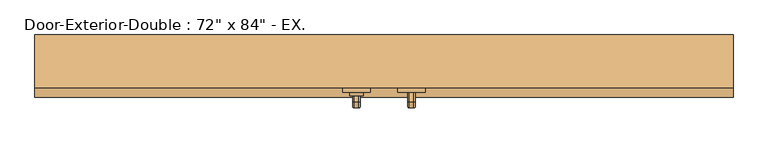
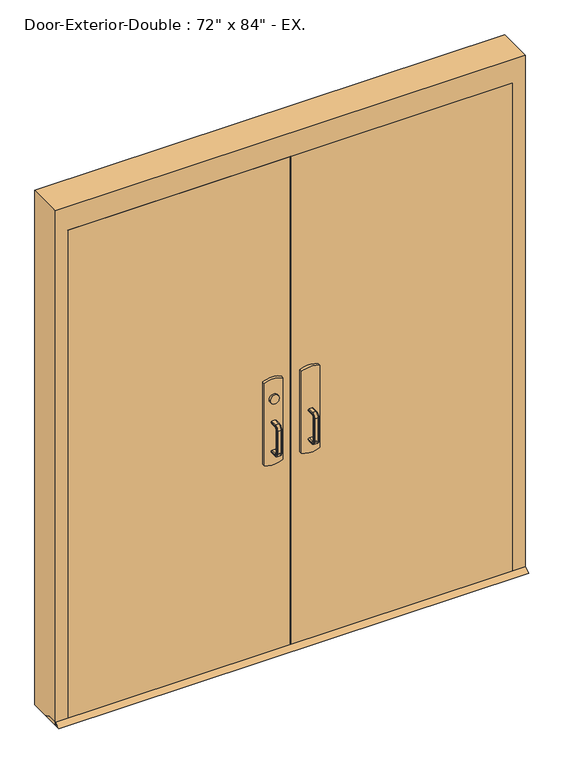
"""IFC4 building model written with IfcOpenShell, lengths in millimetres: door geometry."""

from ifc_helpers import new_model, si_unit, point, frame, frame_2d, origin, place, context, project, spatial, polyline, circle_curve, ellipse_curve, trimmed, segment, composite_curve, outline, extrude, faceted_brep, source, transform, mapped, element, save
from ifc_brep_helpers import plane_surface, cylinder_surface, revolved_surface, advanced_brep


def door_c05566ca(model_context):
    return source(origin(), model_context, "Body", "SolidModel", [
        extrude(outline(polyline([(-575.7333333, -15.875), (-76.2, -15.875), (-76.2, -22.225), (-575.7333333, -22.225), (-575.7333333, -15.875)])), frame((0.0, 0.0, 990.6), z_axis=(0.0, 0.0, 1.0), x_axis=(1.0, 0.0, 0.0)), (0.0, 0.0, 1.0), 50.8),
        advanced_brep(
        [(-12.7, -22.225, 1041.4), (-12.7, -22.225, 990.6), (-76.2, -22.225, 990.6), (-825.5, -22.225, 990.6), (-825.5, -22.225, 1041.4), (-76.2, -22.225, 1041.4), (-825.5, -53.975, 1041.4), (-825.5, -53.975, 990.6), (-76.2, -53.975, 990.6), (-76.2, -53.975, 927.1), (-57.15, -53.975, 908.05), (-31.75, -53.975, 908.05), (-12.7, -53.975, 927.1), (-12.7, -53.975, 1104.9), (-31.75, -53.975, 1123.95), (-57.15, -53.975, 1123.95), (-76.2, -53.975, 1104.9), (-76.2, -53.975, 1041.4), (-76.2, -25.4002467, 1041.4), (-12.7, -25.4002467, 1041.4), (-12.7, -30.4104269, 1104.9), (-12.7, -30.4104269, 927.1), (-12.7, -25.4002467, 990.6), (-76.2, -25.4002467, 990.6), (-76.2, -30.4104269, 1104.9), (-76.2, -30.4104269, 927.1), (-31.75, -31.913481, 1123.95), (-57.15, -31.913481, 1123.95), (-57.15, -31.913481, 908.05), (-31.75, -31.913481, 908.05)],
        [
            (0, 1),
            (1, 2),
            (2, 3),
            (3, 4),
            (4, 5),
            (5, 0),
            (6, 7),
            (7, 8),
            (8, 9),
            (9, 10, circle_curve(frame((-57.15, -53.975, 927.1), z_axis=(0.0, -1.0, 0.0), x_axis=(-1.0, 0.0, 0.0)), 19.05)),
            (10, 11),
            (11, 12, circle_curve(frame((-31.75, -53.975, 927.1), z_axis=(0.0, -1.0, 0.0), x_axis=(-1.0, 0.0, 0.0)), 19.05)),
            (12, 13),
            (13, 14, circle_curve(frame((-31.75, -53.975, 1104.9), z_axis=(0.0, -1.0, 0.0), x_axis=(-1.0, 0.0, 0.0)), 19.05)),
            (14, 15),
            (15, 16, circle_curve(frame((-57.15, -53.975, 1104.9), z_axis=(0.0, -1.0, 0.0), x_axis=(-1.0, 0.0, 0.0)), 19.05)),
            (16, 17),
            (17, 6),
            (4, 6),
            (17, 18),
            (18, 19),
            (19, 0),
            (19, 20),
            (20, 13),
            (12, 21),
            (21, 22),
            (22, 1),
            (7, 3),
            (22, 23),
            (23, 8),
            (16, 24),
            (24, 18),
            (23, 25),
            (25, 9),
            (14, 26),
            (26, 27),
            (27, 15),
            (10, 28),
            (28, 29),
            (29, 11),
            (25, 28, ellipse_curve(frame((-57.15, -30.4104269, 927.1), z_axis=(0.0, -0.9969018152893365, 0.07865602756830282), x_axis=(0.0, 0.07865602756830208, 0.9969018152893365)), 19.1092038, 19.05)),
            (27, 24, ellipse_curve(frame((-57.15, -30.4104269, 1104.9), z_axis=(0.0, -0.9969018152893376, -0.07865602756828934), x_axis=(0.0, 0.078656027568288, -0.9969018152893377)), 19.1092038, 19.05)),
            (20, 26, ellipse_curve(frame((-31.75, -30.4104269, 1104.9), z_axis=(0.0, -0.9969018152893376, -0.07865602756828934), x_axis=(0.0, 0.078656027568288, -0.9969018152893377)), 19.1092038, 19.05)),
            (29, 21, ellipse_curve(frame((-31.75, -30.4104269, 927.1), z_axis=(0.0, -0.9969018152893365, 0.07865602756830282), x_axis=(0.0, 0.07865602756830208, 0.9969018152893365)), 19.1092038, 19.05)),
        ],
        [
            plane_surface(frame((-12.7, -22.225, 1041.4), z_axis=(0.0, 1.0, 0.0), x_axis=(1.0, 0.0, 0.0))),
            plane_surface(frame((-12.7, -53.975, 1041.4), z_axis=(0.0, -1.0, 0.0), x_axis=(-1.0, 0.0, 0.0))),
            plane_surface(frame((-825.5, -22.225, 1041.4), z_axis=(0.0, 0.0, 1.0), x_axis=(0.0, -1.0, 0.0))),
            plane_surface(frame((-12.7, -22.225, 1041.4), z_axis=(1.0, 0.0, 0.0), x_axis=(0.0, -1.0, 0.0))),
            plane_surface(frame((-12.7, -22.225, 990.6), z_axis=(0.0, 0.0, -1.0), x_axis=(0.0, -1.0, 0.0))),
            plane_surface(frame((-825.5, -22.225, 990.6), z_axis=(-1.0, 0.0, 0.0), x_axis=(0.0, -1.0, 0.0))),
            plane_surface(frame((-76.2, -25.4002467, 927.1), z_axis=(-1.0, 0.0, 0.0), x_axis=(0.0, -1.0, 0.0))),
            plane_surface(frame((-57.15, -25.4002467, 1123.95), z_axis=(0.0, 0.0, 1.0), x_axis=(0.0, -1.0, 0.0))),
            plane_surface(frame((-31.75, -25.4002467, 908.05), z_axis=(0.0, 0.0, -1.0), x_axis=(0.0, -1.0, 0.0))),
            cylinder_surface(frame((-57.15, -53.975, 927.1), z_axis=(0.0, 1.0, 0.0), x_axis=(-1.0, 0.0, 0.0)), 19.05),
            cylinder_surface(frame((-57.15, -53.975, 1104.9), z_axis=(0.0, 1.0, 0.0), x_axis=(-1.0, 0.0, 0.0)), 19.05),
            cylinder_surface(frame((-31.75, -53.975, 1104.9), z_axis=(0.0, 1.0, 0.0), x_axis=(-1.0, 0.0, 0.0)), 19.05),
            cylinder_surface(frame((-31.75, -53.975, 927.1), z_axis=(0.0, 1.0, 0.0), x_axis=(-1.0, 0.0, 0.0)), 19.05),
            plane_surface(frame((-76.2, -25.4002467, 1041.4), z_axis=(0.0, 0.9969018152893376, 0.07865602756828934), x_axis=(1.0, 0.0, 0.0))),
            plane_surface(frame((-76.2, -31.913481, 908.05), z_axis=(0.0, 0.9969018152893365, -0.07865602756830282), x_axis=(1.0, 0.0, 0.0))),
        ],
        [
            (0, [[1, 2, 3, 4, 5, 6]]),
            (1, [[7, 8, 9, 10, 11, 12, 13, 14, 15, 16, 17, 18]]),
            (2, [[19, -18, 20, 21, 22, -6, -5]]),
            (3, [[-1, -22, 23, 24, -13, 25, 26, 27]]),
            (4, [[28, -3, -2, -27, 29, 30, -8]]),
            (5, [[-4, -28, -7, -19]]),
            (6, [[-17, 31, 32, -20]]),
            (6, [[-9, -30, 33, 34]]),
            (7, [[-15, 35, 36, 37]]),
            (8, [[-11, 38, 39, 40]]),
            (9, [[-10, -34, 41, -38]]),
            (10, [[-16, -37, 42, -31]]),
            (11, [[-14, -24, 43, -35]]),
            (12, [[-12, -40, 44, -25]]),
            (13, [[-21, -32, -42, -36, -43, -23]]),
            (14, [[-26, -44, -39, -41, -33, -29]]),
        ],
    ),
        extrude(outline(polyline([(-98.425, 12.7), (-53.975, 12.7), (-28.575, 0.0), (-123.825, 0.0), (-98.425, 12.7)])), frame((-965.2, 0.0, 0.0), z_axis=(1.0, 0.0, 0.0), x_axis=(0.0, 1.0, 0.0)), (0.0, 0.0, 1.0), 1930.4),
        extrude(outline(polyline([(575.7333333, -15.875), (575.7333333, -22.225), (76.2, -22.225), (76.2, -15.875), (575.7333333, -15.875)])), frame((0.0, 0.0, 990.6), z_axis=(0.0, 0.0, 1.0), x_axis=(1.0, 0.0, 0.0)), (0.0, 0.0, 1.0), 50.8),
        advanced_brep(
        [(12.7, -22.225, 1041.4), (76.2, -22.225, 1041.4), (825.5, -22.225, 1041.4), (825.5, -22.225, 990.6), (76.2, -22.225, 990.6), (12.7, -22.225, 990.6), (825.5, -53.975, 1041.4), (76.2, -53.975, 1041.4), (76.2, -53.975, 1104.9), (57.15, -53.975, 1123.95), (31.75, -53.975, 1123.95), (12.7, -53.975, 1104.9), (12.7, -53.975, 927.1), (31.75, -53.975, 908.05), (57.15, -53.975, 908.05), (76.2, -53.975, 927.1), (76.2, -53.975, 990.6), (825.5, -53.975, 990.6), (12.7, -25.4002467, 1041.4), (76.2, -25.4002467, 1041.4), (12.7, -25.4002467, 990.6), (12.7, -30.4104269, 927.1), (12.7, -30.4104269, 1104.9), (76.2, -25.4002467, 990.6), (76.2, -30.4104269, 1104.9), (76.2, -30.4104269, 927.1), (57.15, -31.913481, 1123.95), (31.75, -31.913481, 1123.95), (31.75, -31.913481, 908.05), (57.15, -31.913481, 908.05)],
        [
            (0, 1),
            (1, 2),
            (2, 3),
            (3, 4),
            (4, 5),
            (5, 0),
            (6, 7),
            (7, 8),
            (8, 9, circle_curve(frame((57.15, -53.975, 1104.9), z_axis=(0.0, -1.0, 0.0), x_axis=(1.0, 0.0, 0.0)), 19.05)),
            (9, 10),
            (10, 11, circle_curve(frame((31.75, -53.975, 1104.9), z_axis=(0.0, -1.0, 0.0), x_axis=(1.0, 0.0, 0.0)), 19.05)),
            (11, 12),
            (12, 13, circle_curve(frame((31.75, -53.975, 927.1), z_axis=(0.0, -1.0, 0.0), x_axis=(1.0, 0.0, 0.0)), 19.05)),
            (13, 14),
            (14, 15, circle_curve(frame((57.15, -53.975, 927.1), z_axis=(0.0, -1.0, 0.0), x_axis=(1.0, 0.0, 0.0)), 19.05)),
            (15, 16),
            (16, 17),
            (17, 6),
            (0, 18),
            (18, 19),
            (19, 7),
            (6, 2),
            (5, 20),
            (20, 21),
            (21, 12),
            (11, 22),
            (22, 18),
            (16, 23),
            (23, 20),
            (3, 17),
            (19, 24),
            (24, 8),
            (15, 25),
            (25, 23),
            (9, 26),
            (26, 27),
            (27, 10),
            (13, 28),
            (28, 29),
            (29, 14),
            (29, 25, ellipse_curve(frame((57.15, -30.4104269, 927.1), z_axis=(0.0, -0.9969018152893365, 0.07865602756830282), x_axis=(0.0, 0.07865602756830208, 0.9969018152893365)), 19.1092038, 19.05)),
            (24, 26, ellipse_curve(frame((57.15, -30.4104269, 1104.9), z_axis=(0.0, -0.9969018152893376, -0.07865602756828934), x_axis=(0.0, 0.078656027568288, -0.9969018152893377)), 19.1092038, 19.05)),
            (27, 22, ellipse_curve(frame((31.75, -30.4104269, 1104.9), z_axis=(0.0, -0.9969018152893376, -0.07865602756828934), x_axis=(0.0, 0.078656027568288, -0.9969018152893377)), 19.1092038, 19.05)),
            (21, 28, ellipse_curve(frame((31.75, -30.4104269, 927.1), z_axis=(0.0, -0.9969018152893365, 0.07865602756830282), x_axis=(0.0, 0.07865602756830208, 0.9969018152893365)), 19.1092038, 19.05)),
        ],
        [
            plane_surface(frame((12.7, -22.225, 1041.4), z_axis=(0.0, 1.0, 0.0), x_axis=(-1.0, 0.0, 0.0))),
            plane_surface(frame((12.7, -53.975, 1041.4), z_axis=(0.0, -1.0, 0.0), x_axis=(1.0, 0.0, 0.0))),
            plane_surface(frame((825.5, -22.225, 1041.4), z_axis=(0.0, 0.0, 1.0), x_axis=(0.0, -1.0, 0.0))),
            plane_surface(frame((12.7, -22.225, 1041.4), z_axis=(-1.0, 0.0, 0.0), x_axis=(0.0, -1.0, 0.0))),
            plane_surface(frame((12.7, -22.225, 990.6), z_axis=(0.0, 0.0, -1.0), x_axis=(0.0, -1.0, 0.0))),
            plane_surface(frame((825.5, -22.225, 990.6), z_axis=(1.0, 0.0, 0.0), x_axis=(0.0, -1.0, 0.0))),
            plane_surface(frame((76.2, -25.4002467, 927.1), z_axis=(1.0, 0.0, 0.0), x_axis=(0.0, -1.0, 0.0))),
            plane_surface(frame((57.15, -25.4002467, 1123.95), z_axis=(0.0, 0.0, 1.0), x_axis=(0.0, -1.0, 0.0))),
            plane_surface(frame((31.75, -25.4002467, 908.05), z_axis=(0.0, 0.0, -1.0), x_axis=(0.0, -1.0, 0.0))),
            cylinder_surface(frame((57.15, -53.975, 927.1), z_axis=(0.0, 1.0, 0.0), x_axis=(1.0, 0.0, 0.0)), 19.05),
            cylinder_surface(frame((57.15, -53.975, 1104.9), z_axis=(0.0, 1.0, 0.0), x_axis=(1.0, 0.0, 0.0)), 19.05),
            cylinder_surface(frame((31.75, -53.975, 1104.9), z_axis=(0.0, 1.0, 0.0), x_axis=(1.0, 0.0, 0.0)), 19.05),
            cylinder_surface(frame((31.75, -53.975, 927.1), z_axis=(0.0, 1.0, 0.0), x_axis=(1.0, 0.0, 0.0)), 19.05),
            plane_surface(frame((76.2, -25.4002467, 1041.4), z_axis=(0.0, 0.9969018152893376, 0.07865602756828934), x_axis=(-1.0, 0.0, 0.0))),
            plane_surface(frame((76.2, -31.913481, 908.05), z_axis=(0.0, 0.9969018152893365, -0.07865602756830282), x_axis=(-1.0, 0.0, 0.0))),
        ],
        [
            (0, [[1, 2, 3, 4, 5, 6]]),
            (1, [[7, 8, 9, 10, 11, 12, 13, 14, 15, 16, 17, 18]]),
            (2, [[-2, -1, 19, 20, 21, -7, 22]]),
            (3, [[23, 24, 25, -12, 26, 27, -19, -6]]),
            (4, [[-17, 28, 29, -23, -5, -4, 30]]),
            (5, [[-22, -18, -30, -3]]),
            (6, [[-21, 31, 32, -8]]),
            (6, [[33, 34, -28, -16]]),
            (7, [[35, 36, 37, -10]]),
            (8, [[38, 39, 40, -14]]),
            (9, [[-40, 41, -33, -15]]),
            (10, [[-32, 42, -35, -9]]),
            (11, [[-37, 43, -26, -11]]),
            (12, [[-25, 44, -38, -13]]),
            (13, [[-27, -43, -36, -42, -31, -20]]),
            (14, [[-29, -34, -41, -39, -44, -24]]),
        ],
    ),
        advanced_brep(
        [(66.2, -111.125, 1017.190625), (69.771875, -111.125, 1020.7625), (82.628125, -111.125, 1020.7625), (86.2, -111.125, 1017.190625), (86.2, -111.125, 1014.8090406), (82.6284594, -111.125, 1011.2375), (69.771875, -111.125, 1011.2375), (66.2, -111.125, 1014.809375), (66.2, -111.125, 887.809375), (66.2, -111.125, 890.190625), (69.771875, -111.125, 893.7625), (82.6284594, -111.125, 893.7625), (86.2, -111.125, 890.1909594), (86.2, -111.125, 887.809375), (82.628125, -111.125, 884.2375), (69.771875, -111.125, 884.2375), (66.2, -136.525, 1014.809375), (66.2, -148.034375, 1003.3), (66.2, -148.034375, 901.7), (66.2, -136.525, 890.190625), (66.2, -136.525, 887.809375), (66.2, -150.415625, 901.7), (66.2, -150.415625, 1003.3), (66.2, -136.525, 1017.190625), (69.771875, -136.525, 1011.2375), (82.6284594, -136.525, 1011.2375), (86.2, -136.525, 1014.8090406), (86.2, -136.525, 1017.190625), (86.2, -150.415625, 1003.3), (86.2, -150.415625, 901.7), (86.2, -136.525, 887.809375), (86.2, -136.525, 890.1909594), (86.2, -148.0340406, 901.7), (86.2, -148.0340406, 1003.3), (82.628125, -136.525, 1020.7625), (69.771875, -136.525, 1020.7625), (69.771875, -144.4625, 1003.3), (82.6284594, -144.4625, 1003.3), (82.628125, -153.9875, 1003.3), (69.771875, -153.9875, 1003.3), (69.771875, -144.4625, 901.7), (82.6284594, -144.4625, 901.7), (82.628125, -153.9875, 901.7), (69.771875, -153.9875, 901.7), (69.771875, -136.525, 893.7625), (82.6284594, -136.525, 893.7625), (82.628125, -136.525, 884.2375), (69.771875, -136.525, 884.2375)],
        [
            (0, 1, circle_curve(frame((69.771875, -111.125, 1017.190625), z_axis=(0.0, 1.0, 0.0), x_axis=(0.0, 0.0, 1.0)), 3.571875)),
            (1, 2),
            (2, 3, circle_curve(frame((82.628125, -111.125, 1017.190625), z_axis=(0.0, 1.0, 0.0), x_axis=(0.0, 0.0, 1.0)), 3.571875)),
            (3, 4),
            (4, 5, circle_curve(frame((82.6284594, -111.125, 1014.8090406), z_axis=(0.0, 1.0, 0.0), x_axis=(0.0, 0.0, 1.0)), 3.5715406)),
            (5, 6),
            (6, 7, circle_curve(frame((69.771875, -111.125, 1014.809375), z_axis=(0.0, 1.0, 0.0), x_axis=(0.0, 0.0, 1.0)), 3.571875)),
            (7, 0),
            (8, 9),
            (9, 10, circle_curve(frame((69.771875, -111.125, 890.190625), z_axis=(0.0, 1.0, 0.0), x_axis=(0.0, 0.0, -1.0)), 3.571875)),
            (10, 11),
            (11, 12, circle_curve(frame((82.6284594, -111.125, 890.1909594), z_axis=(0.0, 1.0, 0.0), x_axis=(0.0, 0.0, -1.0)), 3.5715406)),
            (12, 13),
            (13, 14, circle_curve(frame((82.628125, -111.125, 887.809375), z_axis=(0.0, 1.0, 0.0), x_axis=(0.0, 0.0, -1.0)), 3.571875)),
            (14, 15),
            (15, 8, circle_curve(frame((69.771875, -111.125, 887.809375), z_axis=(0.0, 1.0, 0.0), x_axis=(0.0, 0.0, -1.0)), 3.571875)),
            (7, 16),
            (16, 17, circle_curve(frame((66.2, -136.525, 1003.3), z_axis=(1.0, 0.0, 0.0), x_axis=(0.0, 0.0, 1.0)), 11.509375)),
            (17, 18),
            (18, 19, circle_curve(frame((66.2, -136.525, 901.7), z_axis=(1.0, 0.0, 0.0), x_axis=(0.0, -1.0, 0.0)), 11.509375)),
            (19, 9),
            (8, 20),
            (20, 21, circle_curve(frame((66.2, -136.525, 901.7), z_axis=(-1.0, 0.0, 0.0), x_axis=(0.0, -1.0, 0.0)), 13.890625)),
            (21, 22),
            (22, 23, circle_curve(frame((66.2, -136.525, 1003.3), z_axis=(-1.0, 0.0, 0.0), x_axis=(0.0, 0.0, 1.0)), 13.890625)),
            (23, 0),
            (6, 24),
            (24, 16, circle_curve(frame((69.771875, -136.525, 1014.809375), z_axis=(0.0, 1.0, 0.0), x_axis=(0.0, 0.0, 1.0)), 3.571875)),
            (5, 25),
            (25, 24),
            (4, 26),
            (26, 25, circle_curve(frame((82.6284594, -136.525, 1014.8090406), z_axis=(0.0, 1.0, 0.0), x_axis=(0.0, 0.0, 1.0)), 3.5715406)),
            (3, 27),
            (27, 28, circle_curve(frame((86.2, -136.525, 1003.3), z_axis=(1.0, 0.0, 0.0), x_axis=(0.0, 0.0, 1.0)), 13.890625)),
            (28, 29),
            (29, 30, circle_curve(frame((86.2, -136.525, 901.7), z_axis=(1.0, 0.0, 0.0), x_axis=(0.0, -1.0, 0.0)), 13.890625)),
            (30, 13),
            (12, 31),
            (31, 32, circle_curve(frame((86.2, -136.525, 901.7), z_axis=(-1.0, 0.0, 0.0), x_axis=(0.0, -1.0, 0.0)), 11.5090406)),
            (32, 33),
            (33, 26, circle_curve(frame((86.2, -136.525, 1003.3), z_axis=(-1.0, 0.0, 0.0), x_axis=(0.0, 0.0, 1.0)), 11.5090406)),
            (2, 34),
            (34, 27, circle_curve(frame((82.628125, -136.525, 1017.190625), z_axis=(0.0, 1.0, 0.0), x_axis=(0.0, 0.0, 1.0)), 3.571875)),
            (1, 35),
            (35, 34),
            (23, 35, circle_curve(frame((69.771875, -136.525, 1017.190625), z_axis=(0.0, 1.0, 0.0), x_axis=(0.0, 0.0, 1.0)), 3.571875)),
            (36, 17, circle_curve(frame((69.771875, -148.034375, 1003.3), z_axis=(0.0, 0.0, 1.0), x_axis=(0.0, -1.0, 0.0)), 3.571875)),
            (24, 36, circle_curve(frame((69.771875, -136.525, 1003.3), z_axis=(1.0, 0.0, 0.0), x_axis=(0.0, 0.0, 1.0)), 7.9375)),
            (37, 36),
            (25, 37, circle_curve(frame((82.6284594, -136.525, 1003.3), z_axis=(1.0, 0.0, 0.0), x_axis=(0.0, 0.0, 1.0)), 7.9375)),
            (33, 37, circle_curve(frame((82.6284594, -148.0340406, 1003.3), z_axis=(0.0, 0.0, 1.0), x_axis=(0.0, -1.0, 0.0)), 3.5715406)),
            (38, 28, circle_curve(frame((82.628125, -150.415625, 1003.3), z_axis=(0.0, 0.0, 1.0), x_axis=(0.0, -1.0, 0.0)), 3.571875)),
            (34, 38, circle_curve(frame((82.628125, -136.525, 1003.3), z_axis=(1.0, 0.0, 0.0), x_axis=(0.0, 0.0, 1.0)), 17.4625)),
            (39, 38),
            (35, 39, circle_curve(frame((69.771875, -136.525, 1003.3), z_axis=(1.0, 0.0, 0.0), x_axis=(0.0, 0.0, 1.0)), 17.4625)),
            (22, 39, circle_curve(frame((69.771875, -150.415625, 1003.3), z_axis=(0.0, 0.0, 1.0), x_axis=(0.0, -1.0, 0.0)), 3.571875)),
            (36, 40),
            (40, 18, circle_curve(frame((69.771875, -148.034375, 901.7), z_axis=(0.0, 0.0, 1.0), x_axis=(0.0, -1.0, 0.0)), 3.571875)),
            (37, 41),
            (41, 40),
            (32, 41, circle_curve(frame((82.6284594, -148.0340406, 901.7), z_axis=(0.0, 0.0, 1.0), x_axis=(0.0, -1.0, 0.0)), 3.5715406)),
            (38, 42),
            (42, 29, circle_curve(frame((82.628125, -150.415625, 901.7), z_axis=(0.0, 0.0, 1.0), x_axis=(0.0, -1.0, 0.0)), 3.571875)),
            (39, 43),
            (43, 42),
            (21, 43, circle_curve(frame((69.771875, -150.415625, 901.7), z_axis=(0.0, 0.0, 1.0), x_axis=(0.0, -1.0, 0.0)), 3.571875)),
            (44, 19, circle_curve(frame((69.771875, -136.525, 890.190625), z_axis=(0.0, -1.0, 0.0), x_axis=(0.0, 0.0, -1.0)), 3.571875)),
            (40, 44, circle_curve(frame((69.771875, -136.525, 901.7), z_axis=(1.0, 0.0, 0.0), x_axis=(0.0, -1.0, 0.0)), 7.9375)),
            (45, 44),
            (41, 45, circle_curve(frame((82.6284594, -136.525, 901.7), z_axis=(1.0, 0.0, 0.0), x_axis=(0.0, -1.0, 0.0)), 7.9375)),
            (31, 45, circle_curve(frame((82.6284594, -136.525, 890.1909594), z_axis=(0.0, -1.0, 0.0), x_axis=(0.0, 0.0, -1.0)), 3.5715406)),
            (46, 30, circle_curve(frame((82.628125, -136.525, 887.809375), z_axis=(0.0, -1.0, 0.0), x_axis=(0.0, 0.0, -1.0)), 3.571875)),
            (42, 46, circle_curve(frame((82.628125, -136.525, 901.7), z_axis=(1.0, 0.0, 0.0), x_axis=(0.0, -1.0, 0.0)), 17.4625)),
            (47, 46),
            (43, 47, circle_curve(frame((69.771875, -136.525, 901.7), z_axis=(1.0, 0.0, 0.0), x_axis=(0.0, -1.0, 0.0)), 17.4625)),
            (20, 47, circle_curve(frame((69.771875, -136.525, 887.809375), z_axis=(0.0, -1.0, 0.0), x_axis=(0.0, 0.0, -1.0)), 3.571875)),
            (44, 10),
            (45, 11),
            (46, 14),
            (47, 15),
        ],
        [
            plane_surface(frame((76.2, -111.125, 1016.0), z_axis=(0.0, 1.0, 0.0), x_axis=(1.0, 0.0, 0.0))),
            plane_surface(frame((76.2, -111.125, 889.0), z_axis=(0.0, 1.0, 0.0), x_axis=(1.0, 0.0, 0.0))),
            plane_surface(frame((66.2, -111.125, 1017.190625), z_axis=(-1.0, 0.0, 0.0), x_axis=(0.0, -1.0, 0.0))),
            cylinder_surface(frame((69.771875, -111.125, 1014.809375), z_axis=(0.0, 1.0, 0.0), x_axis=(0.0, 0.0, 1.0)), 3.571875),
            plane_surface(frame((69.771875, -111.125, 1011.2375), z_axis=(0.0, 0.0, -1.0), x_axis=(0.0, -1.0, 0.0))),
            cylinder_surface(frame((82.6284594, -111.125, 1014.8090406), z_axis=(0.0, 1.0, 0.0), x_axis=(0.0, 0.0, 1.0)), 3.5715406),
            plane_surface(frame((86.2, -111.125, 1014.8090406), z_axis=(1.0, 0.0, 0.0), x_axis=(0.0, -1.0, 0.0))),
            cylinder_surface(frame((82.628125, -111.125, 1017.190625), z_axis=(0.0, 1.0, 0.0), x_axis=(0.0, 0.0, 1.0)), 3.571875),
            plane_surface(frame((82.628125, -111.125, 1020.7625), z_axis=(0.0, 0.0, 1.0), x_axis=(0.0, -1.0, 0.0))),
            cylinder_surface(frame((69.771875, -111.125, 1017.190625), z_axis=(0.0, 1.0, 0.0), x_axis=(0.0, 0.0, 1.0)), 3.571875),
            revolved_surface(trimmed(ellipse_curve(frame((69.771875, -136.525, 1014.809375), z_axis=(0.0, -1.0, 0.0), x_axis=(0.0, 0.0, 1.0)), 3.571875, 3.571875), [point((66.2, -136.525, 1014.809375))], [point((69.771875, -136.525, 1011.2375))], True, "CARTESIAN"), (76.2, -136.525, 1003.3), (-1.0, 0.0, 0.0)),
            revolved_surface(polyline([(69.771875, -136.525, 1011.2375), (82.6284594, -136.525, 1011.2375)]), (76.2, -136.525, 1003.3), (-1.0, 0.0, 0.0)),
            revolved_surface(trimmed(ellipse_curve(frame((82.6284594, -136.525, 1014.8090406), z_axis=(0.0, -1.0, 0.0), x_axis=(0.0, 0.0, 1.0)), 3.5715406, 3.5715406), [point((82.6284594, -136.525, 1011.2375))], [point((86.2, -136.525, 1014.8090406))], True, "CARTESIAN"), (76.2, -136.525, 1003.3), (-1.0, 0.0, 0.0)),
            revolved_surface(trimmed(ellipse_curve(frame((82.628125, -136.525, 1017.190625), z_axis=(0.0, -1.0, 0.0), x_axis=(0.0, 0.0, 1.0)), 3.571875, 3.571875), [point((86.2, -136.525, 1017.190625))], [point((82.628125, -136.525, 1020.7625))], True, "CARTESIAN"), (76.2, -136.525, 1003.3), (-1.0, 0.0, 0.0)),
            cylinder_surface(frame((76.2, -136.525, 1003.3), z_axis=(-1.0, 0.0, 0.0), x_axis=(0.0, 0.0, 1.0)), 17.4625),
            revolved_surface(trimmed(ellipse_curve(frame((69.771875, -136.525, 1017.190625), z_axis=(0.0, -1.0, 0.0), x_axis=(0.0, 0.0, 1.0)), 3.571875, 3.571875), [point((69.771875, -136.525, 1020.7625))], [point((66.2, -136.525, 1017.190625))], True, "CARTESIAN"), (76.2, -136.525, 1003.3), (-1.0, 0.0, 0.0)),
            cylinder_surface(frame((69.771875, -148.034375, 1003.3), z_axis=(0.0, 0.0, 1.0), x_axis=(0.0, -1.0, 0.0)), 3.571875),
            plane_surface(frame((69.771875, -144.4625, 1003.3), z_axis=(0.0, 1.0, 0.0), x_axis=(0.0, 0.0, -1.0))),
            cylinder_surface(frame((82.6284594, -148.0340406, 1003.3), z_axis=(0.0, 0.0, 1.0), x_axis=(0.0, -1.0, 0.0)), 3.5715406),
            cylinder_surface(frame((82.628125, -150.415625, 1003.3), z_axis=(0.0, 0.0, 1.0), x_axis=(0.0, -1.0, 0.0)), 3.571875),
            plane_surface(frame((82.628125, -153.9875, 1003.3), z_axis=(0.0, -1.0, 0.0), x_axis=(0.0, 0.0, -1.0))),
            cylinder_surface(frame((69.771875, -150.415625, 1003.3), z_axis=(0.0, 0.0, 1.0), x_axis=(0.0, -1.0, 0.0)), 3.571875),
            revolved_surface(trimmed(ellipse_curve(frame((69.771875, -148.034375, 901.7), z_axis=(0.0, 0.0, -1.0), x_axis=(0.0, -1.0, 0.0)), 3.571875, 3.571875), [point((66.2, -148.034375, 901.7))], [point((69.771875, -144.4625, 901.7))], True, "CARTESIAN"), (76.2, -136.525, 901.7), (-1.0, 0.0, 0.0)),
            revolved_surface(polyline([(69.771875, -144.4625, 901.7), (82.6284594, -144.4625, 901.7)]), (76.2, -136.525, 901.7), (-1.0, 0.0, 0.0)),
            revolved_surface(trimmed(ellipse_curve(frame((82.6284594, -148.0340406, 901.7), z_axis=(0.0, 0.0, -1.0), x_axis=(0.0, -1.0, 0.0)), 3.5715406, 3.5715406), [point((82.6284594, -144.4625, 901.7))], [point((86.2, -148.0340406, 901.7))], True, "CARTESIAN"), (76.2, -136.525, 901.7), (-1.0, 0.0, 0.0)),
            revolved_surface(trimmed(ellipse_curve(frame((82.628125, -150.415625, 901.7), z_axis=(0.0, 0.0, -1.0), x_axis=(0.0, -1.0, 0.0)), 3.571875, 3.571875), [point((86.2, -150.415625, 901.7))], [point((82.628125, -153.9875, 901.7))], True, "CARTESIAN"), (76.2, -136.525, 901.7), (-1.0, 0.0, 0.0)),
            cylinder_surface(frame((76.2, -136.525, 901.7), z_axis=(-1.0, 0.0, 0.0), x_axis=(0.0, -1.0, 0.0)), 17.4625),
            revolved_surface(trimmed(ellipse_curve(frame((69.771875, -150.415625, 901.7), z_axis=(0.0, 0.0, -1.0), x_axis=(0.0, -1.0, 0.0)), 3.571875, 3.571875), [point((69.771875, -153.9875, 901.7))], [point((66.2, -150.415625, 901.7))], True, "CARTESIAN"), (76.2, -136.525, 901.7), (-1.0, 0.0, 0.0)),
            cylinder_surface(frame((69.771875, -136.525, 890.190625), z_axis=(0.0, -1.0, 0.0), x_axis=(0.0, 0.0, -1.0)), 3.571875),
            plane_surface(frame((69.771875, -136.525, 893.7625), z_axis=(0.0, 0.0, 1.0), x_axis=(0.0, 1.0, 0.0))),
            cylinder_surface(frame((82.6284594, -136.525, 890.1909594), z_axis=(0.0, -1.0, 0.0), x_axis=(0.0, 0.0, -1.0)), 3.5715406),
            cylinder_surface(frame((82.628125, -136.525, 887.809375), z_axis=(0.0, -1.0, 0.0), x_axis=(0.0, 0.0, -1.0)), 3.571875),
            plane_surface(frame((82.628125, -136.525, 884.2375), z_axis=(0.0, 0.0, -1.0), x_axis=(0.0, 1.0, 0.0))),
            cylinder_surface(frame((69.771875, -136.525, 887.809375), z_axis=(0.0, -1.0, 0.0), x_axis=(0.0, 0.0, -1.0)), 3.571875),
        ],
        [
            (0, [[1, 2, 3, 4, 5, 6, 7, 8]]),
            (1, [[9, 10, 11, 12, 13, 14, 15, 16]]),
            (2, [[17, 18, 19, 20, 21, -9, 22, 23, 24, 25, 26, -8]]),
            (3, [[27, 28, -17, -7]]),
            (4, [[29, 30, -27, -6]]),
            (5, [[31, 32, -29, -5]]),
            (6, [[33, 34, 35, 36, 37, -13, 38, 39, 40, 41, -31, -4]]),
            (7, [[42, 43, -33, -3]]),
            (8, [[44, 45, -42, -2]]),
            (9, [[-26, 46, -44, -1]]),
            (10, [[47, -18, -28, 48]]),
            (11, [[49, -48, -30, 50]]),
            (12, [[51, -50, -32, -41]]),
            (13, [[52, -34, -43, 53]]),
            (14, [[54, -53, -45, 55]]),
            (15, [[56, -55, -46, -25]]),
            (16, [[57, 58, -19, -47]]),
            (17, [[59, 60, -57, -49]]),
            (18, [[-40, 61, -59, -51]]),
            (19, [[62, 63, -35, -52]]),
            (20, [[64, 65, -62, -54]]),
            (21, [[-24, 66, -64, -56]]),
            (22, [[67, -20, -58, 68]]),
            (23, [[69, -68, -60, 70]]),
            (24, [[71, -70, -61, -39]]),
            (25, [[72, -36, -63, 73]]),
            (26, [[74, -73, -65, 75]]),
            (27, [[76, -75, -66, -23]]),
            (28, [[77, -10, -21, -67]]),
            (29, [[78, -11, -77, -69]]),
            (30, [[-38, -12, -78, -71]]),
            (31, [[79, -14, -37, -72]]),
            (32, [[80, -15, -79, -74]]),
            (33, [[-22, -16, -80, -76]]),
        ],
    ),
        extrude(outline(composite_curve([segment(trimmed(circle_curve(frame_2d((1113.0338574, 76.2)), 89.3016225), [point((1193.8, 114.3))], [point((1193.8, 38.1))], False, "CARTESIAN"), True, "CONTINUOUS"), segment(polyline([(1193.8, 38.1), (838.2, 38.1)]), True, "CONTINUOUS"), segment(trimmed(circle_curve(frame_2d((918.9661426, 76.2)), 89.3016225), [point((838.2, 38.1))], [point((838.2, 114.3))], False, "CARTESIAN"), True, "CONTINUOUS"), segment(polyline([(838.2, 114.3), (1193.8, 114.3)]), True, "CONTINUOUS")], self_intersect=False)), frame((0.0, -111.125, 0.0), z_axis=(0.0, 1.0, 0.0), x_axis=(0.0, 0.0, 1.0)), (0.0, 0.0, 1.0), 12.7),
        advanced_brep(
        [(-86.2, -111.125, 1017.190625), (-82.628125, -111.125, 1020.7625), (-69.771875, -111.125, 1020.7625), (-66.2, -111.125, 1017.190625), (-66.2, -111.125, 1014.8090406), (-69.7715406, -111.125, 1011.2375), (-82.628125, -111.125, 1011.2375), (-86.2, -111.125, 1014.809375), (-86.2, -111.125, 887.809375), (-86.2, -111.125, 890.190625), (-82.628125, -111.125, 893.7625), (-69.7715406, -111.125, 893.7625), (-66.2, -111.125, 890.1909594), (-66.2, -111.125, 887.809375), (-69.771875, -111.125, 884.2375), (-82.628125, -111.125, 884.2375), (-86.2, -136.525, 1014.809375), (-86.2, -148.034375, 1003.3), (-86.2, -148.034375, 901.7), (-86.2, -136.525, 890.190625), (-86.2, -136.525, 887.809375), (-86.2, -150.415625, 901.7), (-86.2, -150.415625, 1003.3), (-86.2, -136.525, 1017.190625), (-82.628125, -136.525, 1011.2375), (-69.7715406, -136.525, 1011.2375), (-66.2, -136.525, 1014.8090406), (-66.2, -136.525, 1017.190625), (-66.2, -150.415625, 1003.3), (-66.2, -150.415625, 901.7), (-66.2, -136.525, 887.809375), (-66.2, -136.525, 890.1909594), (-66.2, -148.0340406, 901.7), (-66.2, -148.0340406, 1003.3), (-69.771875, -136.525, 1020.7625), (-82.628125, -136.525, 1020.7625), (-82.628125, -144.4625, 1003.3), (-69.7715406, -144.4625, 1003.3), (-69.771875, -153.9875, 1003.3), (-82.628125, -153.9875, 1003.3), (-82.628125, -144.4625, 901.7), (-69.7715406, -144.4625, 901.7), (-69.771875, -153.9875, 901.7), (-82.628125, -153.9875, 901.7), (-82.628125, -136.525, 893.7625), (-69.7715406, -136.525, 893.7625), (-69.771875, -136.525, 884.2375), (-82.628125, -136.525, 884.2375)],
        [
            (0, 1, circle_curve(frame((-82.628125, -111.125, 1017.190625), z_axis=(0.0, 1.0, 0.0), x_axis=(0.0, 0.0, 1.0)), 3.571875)),
            (1, 2),
            (2, 3, circle_curve(frame((-69.771875, -111.125, 1017.190625), z_axis=(0.0, 1.0, 0.0), x_axis=(0.0, 0.0, 1.0)), 3.571875)),
            (3, 4),
            (4, 5, circle_curve(frame((-69.7715406, -111.125, 1014.8090406), z_axis=(0.0, 1.0, 0.0), x_axis=(0.0, 0.0, 1.0)), 3.5715406)),
            (5, 6),
            (6, 7, circle_curve(frame((-82.628125, -111.125, 1014.809375), z_axis=(0.0, 1.0, 0.0), x_axis=(0.0, 0.0, 1.0)), 3.571875)),
            (7, 0),
            (8, 9),
            (9, 10, circle_curve(frame((-82.628125, -111.125, 890.190625), z_axis=(0.0, 1.0, 0.0), x_axis=(0.0, 0.0, -1.0)), 3.571875)),
            (10, 11),
            (11, 12, circle_curve(frame((-69.7715406, -111.125, 890.1909594), z_axis=(0.0, 1.0, 0.0), x_axis=(0.0, 0.0, -1.0)), 3.5715406)),
            (12, 13),
            (13, 14, circle_curve(frame((-69.771875, -111.125, 887.809375), z_axis=(0.0, 1.0, 0.0), x_axis=(0.0, 0.0, -1.0)), 3.571875)),
            (14, 15),
            (15, 8, circle_curve(frame((-82.628125, -111.125, 887.809375), z_axis=(0.0, 1.0, 0.0), x_axis=(0.0, 0.0, -1.0)), 3.571875)),
            (7, 16),
            (16, 17, circle_curve(frame((-86.2, -136.525, 1003.3), z_axis=(1.0, 0.0, 0.0), x_axis=(0.0, 0.0, 1.0)), 11.509375)),
            (17, 18),
            (18, 19, circle_curve(frame((-86.2, -136.525, 901.7), z_axis=(1.0, 0.0, 0.0), x_axis=(0.0, -1.0, 0.0)), 11.509375)),
            (19, 9),
            (8, 20),
            (20, 21, circle_curve(frame((-86.2, -136.525, 901.7), z_axis=(-1.0, 0.0, 0.0), x_axis=(0.0, -1.0, 0.0)), 13.890625)),
            (21, 22),
            (22, 23, circle_curve(frame((-86.2, -136.525, 1003.3), z_axis=(-1.0, 0.0, 0.0), x_axis=(0.0, 0.0, 1.0)), 13.890625)),
            (23, 0),
            (6, 24),
            (24, 16, circle_curve(frame((-82.628125, -136.525, 1014.809375), z_axis=(0.0, 1.0, 0.0), x_axis=(0.0, 0.0, 1.0)), 3.571875)),
            (5, 25),
            (25, 24),
            (4, 26),
            (26, 25, circle_curve(frame((-69.7715406, -136.525, 1014.8090406), z_axis=(0.0, 1.0, 0.0), x_axis=(0.0, 0.0, 1.0)), 3.5715406)),
            (3, 27),
            (27, 28, circle_curve(frame((-66.2, -136.525, 1003.3), z_axis=(1.0, 0.0, 0.0), x_axis=(0.0, 0.0, 1.0)), 13.890625)),
            (28, 29),
            (29, 30, circle_curve(frame((-66.2, -136.525, 901.7), z_axis=(1.0, 0.0, 0.0), x_axis=(0.0, -1.0, 0.0)), 13.890625)),
            (30, 13),
            (12, 31),
            (31, 32, circle_curve(frame((-66.2, -136.525, 901.7), z_axis=(-1.0, 0.0, 0.0), x_axis=(0.0, -1.0, 0.0)), 11.5090406)),
            (32, 33),
            (33, 26, circle_curve(frame((-66.2, -136.525, 1003.3), z_axis=(-1.0, 0.0, 0.0), x_axis=(0.0, 0.0, 1.0)), 11.5090406)),
            (2, 34),
            (34, 27, circle_curve(frame((-69.771875, -136.525, 1017.190625), z_axis=(0.0, 1.0, 0.0), x_axis=(0.0, 0.0, 1.0)), 3.571875)),
            (1, 35),
            (35, 34),
            (23, 35, circle_curve(frame((-82.628125, -136.525, 1017.190625), z_axis=(0.0, 1.0, 0.0), x_axis=(0.0, 0.0, 1.0)), 3.571875)),
            (36, 17, circle_curve(frame((-82.628125, -148.034375, 1003.3), z_axis=(0.0, 0.0, 1.0), x_axis=(0.0, -1.0, 0.0)), 3.571875)),
            (24, 36, circle_curve(frame((-82.628125, -136.525, 1003.3), z_axis=(1.0, 0.0, 0.0), x_axis=(0.0, 0.0, 1.0)), 7.9375)),
            (37, 36),
            (25, 37, circle_curve(frame((-69.7715406, -136.525, 1003.3), z_axis=(1.0, 0.0, 0.0), x_axis=(0.0, 0.0, 1.0)), 7.9375)),
            (33, 37, circle_curve(frame((-69.7715406, -148.0340406, 1003.3), z_axis=(0.0, 0.0, 1.0), x_axis=(0.0, -1.0, 0.0)), 3.5715406)),
            (38, 28, circle_curve(frame((-69.771875, -150.415625, 1003.3), z_axis=(0.0, 0.0, 1.0), x_axis=(0.0, -1.0, 0.0)), 3.571875)),
            (34, 38, circle_curve(frame((-69.771875, -136.525, 1003.3), z_axis=(1.0, 0.0, 0.0), x_axis=(0.0, 0.0, 1.0)), 17.4625)),
            (39, 38),
            (35, 39, circle_curve(frame((-82.628125, -136.525, 1003.3), z_axis=(1.0, 0.0, 0.0), x_axis=(0.0, 0.0, 1.0)), 17.4625)),
            (22, 39, circle_curve(frame((-82.628125, -150.415625, 1003.3), z_axis=(0.0, 0.0, 1.0), x_axis=(0.0, -1.0, 0.0)), 3.571875)),
            (36, 40),
            (40, 18, circle_curve(frame((-82.628125, -148.034375, 901.7), z_axis=(0.0, 0.0, 1.0), x_axis=(0.0, -1.0, 0.0)), 3.571875)),
            (37, 41),
            (41, 40),
            (32, 41, circle_curve(frame((-69.7715406, -148.0340406, 901.7), z_axis=(0.0, 0.0, 1.0), x_axis=(0.0, -1.0, 0.0)), 3.5715406)),
            (38, 42),
            (42, 29, circle_curve(frame((-69.771875, -150.415625, 901.7), z_axis=(0.0, 0.0, 1.0), x_axis=(0.0, -1.0, 0.0)), 3.571875)),
            (39, 43),
            (43, 42),
            (21, 43, circle_curve(frame((-82.628125, -150.415625, 901.7), z_axis=(0.0, 0.0, 1.0), x_axis=(0.0, -1.0, 0.0)), 3.571875)),
            (44, 19, circle_curve(frame((-82.628125, -136.525, 890.190625), z_axis=(0.0, -1.0, 0.0), x_axis=(0.0, 0.0, -1.0)), 3.571875)),
            (40, 44, circle_curve(frame((-82.628125, -136.525, 901.7), z_axis=(1.0, 0.0, 0.0), x_axis=(0.0, -1.0, 0.0)), 7.9375)),
            (45, 44),
            (41, 45, circle_curve(frame((-69.7715406, -136.525, 901.7), z_axis=(1.0, 0.0, 0.0), x_axis=(0.0, -1.0, 0.0)), 7.9375)),
            (31, 45, circle_curve(frame((-69.7715406, -136.525, 890.1909594), z_axis=(0.0, -1.0, 0.0), x_axis=(0.0, 0.0, -1.0)), 3.5715406)),
            (46, 30, circle_curve(frame((-69.771875, -136.525, 887.809375), z_axis=(0.0, -1.0, 0.0), x_axis=(0.0, 0.0, -1.0)), 3.571875)),
            (42, 46, circle_curve(frame((-69.771875, -136.525, 901.7), z_axis=(1.0, 0.0, 0.0), x_axis=(0.0, -1.0, 0.0)), 17.4625)),
            (47, 46),
            (43, 47, circle_curve(frame((-82.628125, -136.525, 901.7), z_axis=(1.0, 0.0, 0.0), x_axis=(0.0, -1.0, 0.0)), 17.4625)),
            (20, 47, circle_curve(frame((-82.628125, -136.525, 887.809375), z_axis=(0.0, -1.0, 0.0), x_axis=(0.0, 0.0, -1.0)), 3.571875)),
            (44, 10),
            (45, 11),
            (46, 14),
            (47, 15),
        ],
        [
            plane_surface(frame((-76.2, -111.125, 1016.0), z_axis=(0.0, 1.0, 0.0), x_axis=(1.0, 0.0, 0.0))),
            plane_surface(frame((-76.2, -111.125, 889.0), z_axis=(0.0, 1.0, 0.0), x_axis=(1.0, 0.0, 0.0))),
            plane_surface(frame((-86.2, -111.125, 1017.190625), z_axis=(-1.0, 0.0, 0.0), x_axis=(0.0, -1.0, 0.0))),
            cylinder_surface(frame((-82.628125, -111.125, 1014.809375), z_axis=(0.0, 1.0, 0.0), x_axis=(0.0, 0.0, 1.0)), 3.571875),
            plane_surface(frame((-82.628125, -111.125, 1011.2375), z_axis=(0.0, 0.0, -1.0), x_axis=(0.0, -1.0, 0.0))),
            cylinder_surface(frame((-69.7715406, -111.125, 1014.8090406), z_axis=(0.0, 1.0, 0.0), x_axis=(0.0, 0.0, 1.0)), 3.5715406),
            plane_surface(frame((-66.2, -111.125, 1014.8090406), z_axis=(1.0, 0.0, 0.0), x_axis=(0.0, -1.0, 0.0))),
            cylinder_surface(frame((-69.771875, -111.125, 1017.190625), z_axis=(0.0, 1.0, 0.0), x_axis=(0.0, 0.0, 1.0)), 3.571875),
            plane_surface(frame((-69.771875, -111.125, 1020.7625), z_axis=(0.0, 0.0, 1.0), x_axis=(0.0, -1.0, 0.0))),
            cylinder_surface(frame((-82.628125, -111.125, 1017.190625), z_axis=(0.0, 1.0, 0.0), x_axis=(0.0, 0.0, 1.0)), 3.571875),
            revolved_surface(trimmed(ellipse_curve(frame((-82.628125, -136.525, 1014.809375), z_axis=(0.0, -1.0, 0.0), x_axis=(0.0, 0.0, 1.0)), 3.571875, 3.571875), [point((-86.2, -136.525, 1014.809375))], [point((-82.628125, -136.525, 1011.2375))], True, "CARTESIAN"), (-76.2, -136.525, 1003.3), (-1.0, 0.0, 0.0)),
            revolved_surface(polyline([(-82.628125, -136.525, 1011.2375), (-69.7715406, -136.525, 1011.2375)]), (-76.2, -136.525, 1003.3), (-1.0, 0.0, 0.0)),
            revolved_surface(trimmed(ellipse_curve(frame((-69.7715406, -136.525, 1014.8090406), z_axis=(0.0, -1.0, 0.0), x_axis=(0.0, 0.0, 1.0)), 3.5715406, 3.5715406), [point((-69.7715406, -136.525, 1011.2375))], [point((-66.2, -136.525, 1014.8090406))], True, "CARTESIAN"), (-76.2, -136.525, 1003.3), (-1.0, 0.0, 0.0)),
            revolved_surface(trimmed(ellipse_curve(frame((-69.771875, -136.525, 1017.190625), z_axis=(0.0, -1.0, 0.0), x_axis=(0.0, 0.0, 1.0)), 3.571875, 3.571875), [point((-66.2, -136.525, 1017.190625))], [point((-69.771875, -136.525, 1020.7625))], True, "CARTESIAN"), (-76.2, -136.525, 1003.3), (-1.0, 0.0, 0.0)),
            cylinder_surface(frame((-76.2, -136.525, 1003.3), z_axis=(-1.0, 0.0, 0.0), x_axis=(0.0, 0.0, 1.0)), 17.4625),
            revolved_surface(trimmed(ellipse_curve(frame((-82.628125, -136.525, 1017.190625), z_axis=(0.0, -1.0, 0.0), x_axis=(0.0, 0.0, 1.0)), 3.571875, 3.571875), [point((-82.628125, -136.525, 1020.7625))], [point((-86.2, -136.525, 1017.190625))], True, "CARTESIAN"), (-76.2, -136.525, 1003.3), (-1.0, 0.0, 0.0)),
            cylinder_surface(frame((-82.628125, -148.034375, 1003.3), z_axis=(0.0, 0.0, 1.0), x_axis=(0.0, -1.0, 0.0)), 3.571875),
            plane_surface(frame((-82.628125, -144.4625, 1003.3), z_axis=(0.0, 1.0, 0.0), x_axis=(0.0, 0.0, -1.0))),
            cylinder_surface(frame((-69.7715406, -148.0340406, 1003.3), z_axis=(0.0, 0.0, 1.0), x_axis=(0.0, -1.0, 0.0)), 3.5715406),
            cylinder_surface(frame((-69.771875, -150.415625, 1003.3), z_axis=(0.0, 0.0, 1.0), x_axis=(0.0, -1.0, 0.0)), 3.571875),
            plane_surface(frame((-69.771875, -153.9875, 1003.3), z_axis=(0.0, -1.0, 0.0), x_axis=(0.0, 0.0, -1.0))),
            cylinder_surface(frame((-82.628125, -150.415625, 1003.3), z_axis=(0.0, 0.0, 1.0), x_axis=(0.0, -1.0, 0.0)), 3.571875),
            revolved_surface(trimmed(ellipse_curve(frame((-82.628125, -148.034375, 901.7), z_axis=(0.0, 0.0, -1.0), x_axis=(0.0, -1.0, 0.0)), 3.571875, 3.571875), [point((-86.2, -148.034375, 901.7))], [point((-82.628125, -144.4625, 901.7))], True, "CARTESIAN"), (-76.2, -136.525, 901.7), (-1.0, 0.0, 0.0)),
            revolved_surface(polyline([(-82.628125, -144.4625, 901.7), (-69.7715406, -144.4625, 901.7)]), (-76.2, -136.525, 901.7), (-1.0, 0.0, 0.0)),
            revolved_surface(trimmed(ellipse_curve(frame((-69.7715406, -148.0340406, 901.7), z_axis=(0.0, 0.0, -1.0), x_axis=(0.0, -1.0, 0.0)), 3.5715406, 3.5715406), [point((-69.7715406, -144.4625, 901.7))], [point((-66.2, -148.0340406, 901.7))], True, "CARTESIAN"), (-76.2, -136.525, 901.7), (-1.0, 0.0, 0.0)),
            revolved_surface(trimmed(ellipse_curve(frame((-69.771875, -150.415625, 901.7), z_axis=(0.0, 0.0, -1.0), x_axis=(0.0, -1.0, 0.0)), 3.571875, 3.571875), [point((-66.2, -150.415625, 901.7))], [point((-69.771875, -153.9875, 901.7))], True, "CARTESIAN"), (-76.2, -136.525, 901.7), (-1.0, 0.0, 0.0)),
            cylinder_surface(frame((-76.2, -136.525, 901.7), z_axis=(-1.0, 0.0, 0.0), x_axis=(0.0, -1.0, 0.0)), 17.4625),
            revolved_surface(trimmed(ellipse_curve(frame((-82.628125, -150.415625, 901.7), z_axis=(0.0, 0.0, -1.0), x_axis=(0.0, -1.0, 0.0)), 3.571875, 3.571875), [point((-82.628125, -153.9875, 901.7))], [point((-86.2, -150.415625, 901.7))], True, "CARTESIAN"), (-76.2, -136.525, 901.7), (-1.0, 0.0, 0.0)),
            cylinder_surface(frame((-82.628125, -136.525, 890.190625), z_axis=(0.0, -1.0, 0.0), x_axis=(0.0, 0.0, -1.0)), 3.571875),
            plane_surface(frame((-82.628125, -136.525, 893.7625), z_axis=(0.0, 0.0, 1.0), x_axis=(0.0, 1.0, 0.0))),
            cylinder_surface(frame((-69.7715406, -136.525, 890.1909594), z_axis=(0.0, -1.0, 0.0), x_axis=(0.0, 0.0, -1.0)), 3.5715406),
            cylinder_surface(frame((-69.771875, -136.525, 887.809375), z_axis=(0.0, -1.0, 0.0), x_axis=(0.0, 0.0, -1.0)), 3.571875),
            plane_surface(frame((-69.771875, -136.525, 884.2375), z_axis=(0.0, 0.0, -1.0), x_axis=(0.0, 1.0, 0.0))),
            cylinder_surface(frame((-82.628125, -136.525, 887.809375), z_axis=(0.0, -1.0, 0.0), x_axis=(0.0, 0.0, -1.0)), 3.571875),
        ],
        [
            (0, [[1, 2, 3, 4, 5, 6, 7, 8]]),
            (1, [[9, 10, 11, 12, 13, 14, 15, 16]]),
            (2, [[17, 18, 19, 20, 21, -9, 22, 23, 24, 25, 26, -8]]),
            (3, [[27, 28, -17, -7]]),
            (4, [[29, 30, -27, -6]]),
            (5, [[31, 32, -29, -5]]),
            (6, [[33, 34, 35, 36, 37, -13, 38, 39, 40, 41, -31, -4]]),
            (7, [[42, 43, -33, -3]]),
            (8, [[44, 45, -42, -2]]),
            (9, [[-26, 46, -44, -1]]),
            (10, [[47, -18, -28, 48]]),
            (11, [[49, -48, -30, 50]]),
            (12, [[51, -50, -32, -41]]),
            (13, [[52, -34, -43, 53]]),
            (14, [[54, -53, -45, 55]]),
            (15, [[56, -55, -46, -25]]),
            (16, [[57, 58, -19, -47]]),
            (17, [[59, 60, -57, -49]]),
            (18, [[-40, 61, -59, -51]]),
            (19, [[62, 63, -35, -52]]),
            (20, [[64, 65, -62, -54]]),
            (21, [[-24, 66, -64, -56]]),
            (22, [[67, -20, -58, 68]]),
            (23, [[69, -68, -60, 70]]),
            (24, [[71, -70, -61, -39]]),
            (25, [[72, -36, -63, 73]]),
            (26, [[74, -73, -65, 75]]),
            (27, [[76, -75, -66, -23]]),
            (28, [[77, -10, -21, -67]]),
            (29, [[78, -11, -77, -69]]),
            (30, [[-38, -12, -78, -71]]),
            (31, [[79, -14, -37, -72]]),
            (32, [[80, -15, -79, -74]]),
            (33, [[-22, -16, -80, -76]]),
        ],
    ),
        extrude(outline(composite_curve([segment(trimmed(circle_curve(frame_2d((1117.6, -76.2)), 19.0), [point((1117.6, -95.2))], [point((1117.6, -57.2))], False, "CARTESIAN"), True, "CONTINUOUS"), segment(trimmed(circle_curve(frame_2d((1117.6, -76.2)), 19.0), [point((1117.6, -57.2))], [point((1117.6, -95.2))], False, "CARTESIAN"), True, "CONTINUOUS")], self_intersect=False)), frame((0.0, -119.85625, 0.0), z_axis=(0.0, 1.0, 0.0), x_axis=(0.0, 0.0, 1.0)), (0.0, 0.0, 1.0), 8.73125),
        extrude(outline(composite_curve([segment(trimmed(circle_curve(frame_2d((1113.0338574, -76.2)), 89.3016225), [point((1193.8, -38.1))], [point((1193.8, -114.3))], False, "CARTESIAN"), True, "CONTINUOUS"), segment(polyline([(1193.8, -114.3), (838.2, -114.3)]), True, "CONTINUOUS"), segment(trimmed(circle_curve(frame_2d((918.9661426, -76.2)), 89.3016225), [point((838.2, -114.3))], [point((838.2, -38.1))], False, "CARTESIAN"), True, "CONTINUOUS"), segment(polyline([(838.2, -38.1), (1193.8, -38.1)]), True, "CONTINUOUS")], self_intersect=False)), frame((0.0, -111.125, 0.0), z_axis=(0.0, 1.0, 0.0), x_axis=(0.0, 0.0, 1.0)), (0.0, 0.0, 1.0), 12.7),
        faceted_brep([(914.4, -49.2125, 0.0), (898.525, -49.2125, 0.0), (898.525, -1.5875, 0.0), (914.4, -1.5875, 0.0), (914.4, 47.625, 0.0), (965.2, 47.625, 0.0), (965.2, -98.425, 0.0), (914.4, -98.425, 0.0), (914.4, -98.425, 2133.6), (914.4, -49.2125, 2133.6), (965.2, -98.425, 2235.2), (-965.2, -98.425, 2235.2), (-965.2, -98.425, 0.0), (-914.4, -98.425, 0.0), (-914.4, -98.425, 2133.6), (965.2, 47.625, 2235.2), (914.4, 47.625, 2133.6), (-914.4, 47.625, 2133.6), (-914.4, 47.625, 0.0), (-965.2, 47.625, 0.0), (-965.2, 47.625, 2235.2), (914.4, -1.5875, 2133.6), (898.525, -1.5875, 2117.725), (-898.525, -1.5875, 2117.725), (-898.525, -1.5875, 0.0), (-914.4, -1.5875, 0.0), (-914.4, -1.5875, 2133.6), (898.525, -49.2125, 2117.725), (-914.4, -49.2125, 2133.6), (-914.4, -49.2125, 0.0), (-898.525, -49.2125, 0.0), (-898.525, -49.2125, 2117.725)], [[[0, 1, 2, 3, 4, 5, 6, 7]], [[7, 8, 9, 0]], [[6, 10, 11, 12, 13, 14, 8, 7]], [[5, 15, 10, 6]], [[4, 16, 17, 18, 19, 20, 15, 5]], [[3, 21, 16, 4]], [[2, 22, 23, 24, 25, 26, 21, 3]], [[1, 27, 22, 2]], [[0, 9, 28, 29, 30, 31, 27, 1]], [[8, 14, 28, 9]], [[16, 21, 26, 17]], [[22, 27, 31, 23]], [[12, 19, 18, 25, 24, 30, 29, 13]], [[13, 29, 28, 14]], [[11, 20, 19, 12]], [[17, 26, 25, 18]], [[23, 31, 30, 24]], [[15, 20, 11, 10]]]),
        extrude(outline(polyline([(914.4, -53.975), (914.4, -98.425), (1.5875, -98.425), (1.5875, -53.975), (914.4, -53.975)])), frame((0.0, 0.0, 12.7), z_axis=(0.0, 0.0, 1.0), x_axis=(1.0, 0.0, 0.0)), (0.0, 0.0, 1.0), 2120.9),
        extrude(outline(polyline([(-1.5875, -53.975), (-1.5875, -98.425), (-914.4, -98.425), (-914.4, -53.975), (-1.5875, -53.975)])), frame((0.0, 0.0, 12.7), z_axis=(0.0, 0.0, 1.0), x_axis=(1.0, 0.0, 0.0)), (0.0, 0.0, 1.0), 2120.9),
    ])


if __name__ == "__main__":
    model = new_model("IFC4")
    model_context = context("Model", 3, world=origin())
    ifc_project = project(units=[si_unit("LENGTHUNIT", "METRE", prefix="MILLI")], contexts=[model_context])
    site = spatial("IfcSite", under=ifc_project)
    building = spatial("IfcBuilding", under=site)
    placement = place(None, origin())
    door_shape = door_c05566ca(model_context)
    element("IfcDoor", 1, ObjectType="Door-Exterior-Double : 72\" x 84\" - EX.", at=placement, inside=building, context=model_context, shape_type="MappedRepresentation", body=[
        mapped(door_shape, transform((0.0, 0.0, 0.0), x_axis=(1.0, 0.0, 0.0), y_axis=(0.0, 1.0, 0.0), z_axis=(0.0, 0.0, 1.0))),
    ])
    save(model, "model.ifc")

# Revit data of these elements
# Type "Door-Exterior-Double : 72\" x 84\" - EX."
#   Type Mark = "EX-1"
#   Assembly Code = "B2030200"
#   Analytic Construction = "Metal"
#   Threshold Length [instance default] = 6' - 4"
#   Threshold Offset [instance default] = 0' - 0 1/2"
#   Thickness = 0' - 1 3/4"
#   Thermal Resistance (R) = 0.270118 (m²·K)/W
#   Swing Angle [instance default] = 90.00°
#   Strike Height = 3' - 4"
#   SinglePanelWidth = 3' - 0"
#   Rough Width [instance default] = 6' - 4"
#   Rough Height [instance default] = 7' - 4"
#   MFOpeningHeight [instance default] = 0' - 4"
#   MFOpeningWidth [instance default] = 0' - 4"
#   Inset Calculate [instance default] = 0' - 4"
#   Masonry Inset [instance default] = 0' - 1"
#   Height = 7' - 0"
#   Width = 6' - 0"
#   Heat Transfer Coefficient (U) = 3.70223 W/(m²·K)
#   Masonry Frame Depth = 0' - 5 3/4"
#   Threshold [instance default] = yes
#   Masonry Frame [instance default] = yes
#   Function = 1
#   Dry Wall Frame [instance default] = no
#   Threshold Material = Cherry
#   Panic Bar Material = Metal - Stainless Steel
#   Panel Material = Metal - Painted - Grey
#   Frame Material = Metal - Painted - Grey
#   Exterior Pull Material = Metal - Stainless Steel
#   Visual Light Transmittance = 0
#   Solar Heat Gain Coefficient = 0
#   Wall Closure = (empty or 0)
# Element 1 (IfcDoor, "Door-Exterior-Double : 72\" x 84\" - EX.")
#   Materials on its faces: "Metal - Stainless Steel", "Metal - Painted - Grey", "Cherry"
# Materials
#   "Cherry": class "Wood", colour RGB 154 107 61, transparency 0, Description = "Prunus Serotina", Cost = 0
#   "Metal - Stainless Steel": class "Metal", colour RGB 247 247 247, transparency 0
#   "Metal - Painted - Grey": class "Paint", colour RGB 104 104 104, transparency 0
